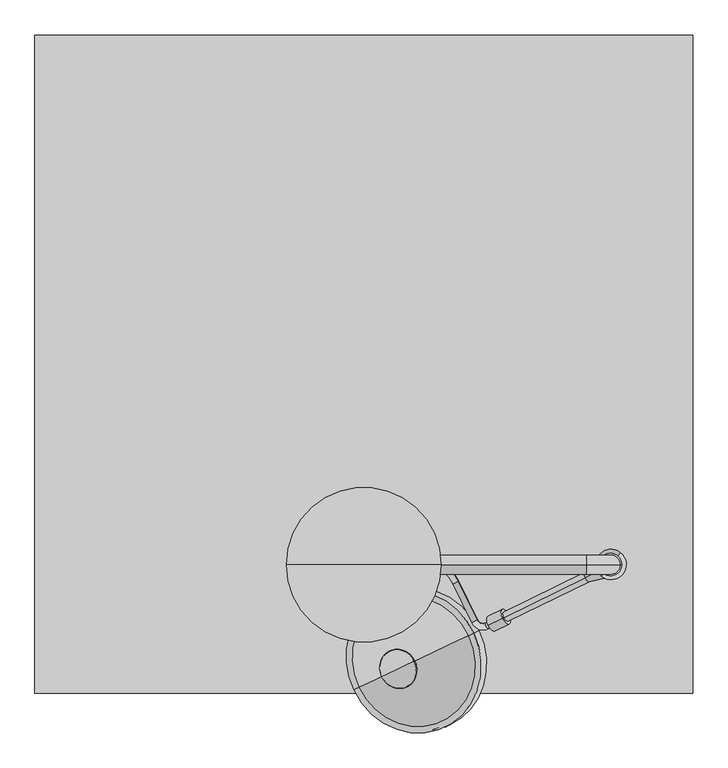
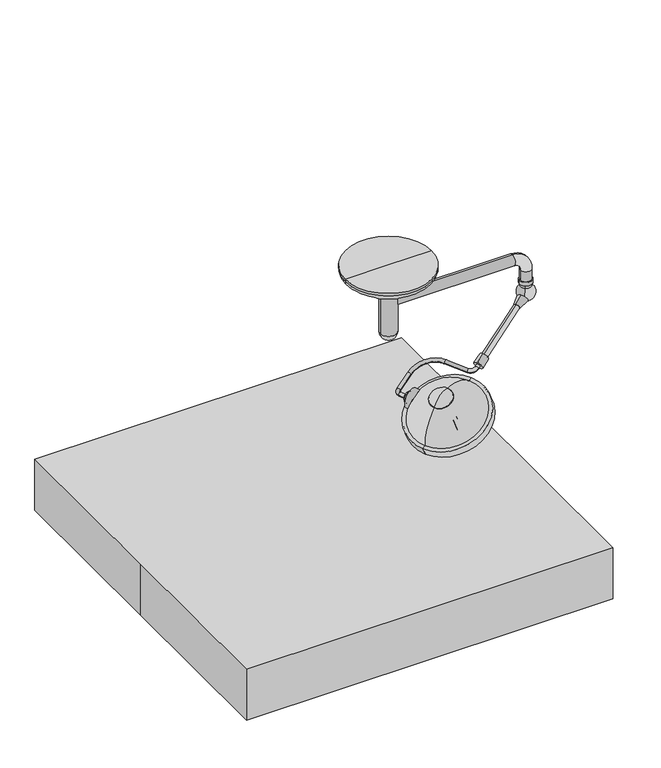
"""IFC4 building model written with IfcOpenShell, lengths in millimetres: proxy geometry, M7485 - Light, Surg, Ceiling Mtd, Dual, Equal Dia Heads : M7485 - Light, Surg, Ceiling Mtd, Dual, Equal Dia Heads."""

from ifc_helpers import new_model, si_unit, point, frame, frame_2d, origin, origin_with_axes, origin_2d, place, context, project, spatial, polyline, circle_curve, ellipse_curve, trimmed, segment, composite_curve, outline, extrude, source, transform, mapped, element, save
from ifc_brep_helpers import plane_surface, cylinder_surface, revolved_surface, advanced_brep


def specialty_equipment_7f5e032a(model_context):
    return source(origin(), model_context, "Body", "SolidModel", [
        advanced_brep(
        [(51.3241797, -908.0178384, 1699.7604265), (72.1798458, -897.8458503, 1710.0915373), (51.503984, -855.4540515, 1710.0915373), (30.6483179, -865.6260395, 1699.7604265), (56.3645035, -838.953373, 1715.2570926), (45.2298764, -816.1240043, 1715.2570926), (159.8794514, -788.4657596, 1766.5344952), (148.7448243, -765.6363908, 1766.5344952), (351.8212111, -864.410044, 1828.5211596), (372.6768772, -854.238056, 1838.8522704), (426.0821694, -1016.6675722, 1828.5211596), (446.9378356, -1006.4955842, 1838.8522704), (490.062756, -1041.9823337, 1849.1833811), (478.9281288, -1019.1529649, 1849.1833811), (557.8921303, -980.6396481, 1888.2991704), (569.0267574, -1003.4690168, 1888.2991704)],
        [
            (0, 1, circle_curve(frame((61.7520127, -902.9318443, 1704.9259819), z_axis=(0.4383711467890926, -0.8987940462991595, 0.0), x_axis=(0.8210892183528103, 0.4004719699107539, 0.4067366430758007)), 12.7)),
            (1, 0, circle_curve(frame((61.7520127, -902.9318443, 1704.9259819), z_axis=(0.4383711467890926, -0.8987940462991595, 0.0), x_axis=(0.8210892183528103, 0.4004719699107539, 0.4067366430758007)), 12.7)),
            (1, 2),
            (2, 3, circle_curve(frame((41.0761509, -860.5400455, 1704.9259819), z_axis=(0.4383711467890926, -0.8987940462991595, 0.0), x_axis=(0.8210892183528103, 0.4004719699107539, 0.4067366430758007)), 12.7)),
            (3, 0),
            (3, 2, circle_curve(frame((41.0761509, -860.5400455, 1704.9259819), z_axis=(0.4383711467890926, -0.8987940462991595, 0.0), x_axis=(0.8210892183528103, 0.4004719699107539, 0.4067366430758007)), 12.7)),
            (4, 5, circle_curve(frame((50.79719, -827.5386887, 1715.2570926), z_axis=(-0.8210892183528203, -0.40047196991073386, -0.4067366430758003), x_axis=(0.4383711467890744, -0.8987940462991688, 0.0)), 12.7)),
            (5, 3, circle_curve(frame((61.9318171, -850.3680574, 1715.2570926), z_axis=(-0.36557247320823616, -0.17830160866628347, 0.9135454576426008), x_axis=(-0.8210892183528108, -0.40047196991075346, -0.40673664307580043)), 38.1)),
            (2, 4, circle_curve(frame((61.9318171, -850.3680574, 1715.2570926), z_axis=(0.36557247320823616, 0.17830160866628347, -0.9135454576426008), x_axis=(-0.8210892183528108, -0.40047196991075346, -0.40673664307580043)), 12.7)),
            (5, 4, circle_curve(frame((50.79719, -827.5386887, 1715.2570926), z_axis=(-0.8210892183528095, -0.40047196991075623, -0.4067366430758003), x_axis=(0.43837114678909483, -0.8987940462991588, 0.0)), 12.7)),
            (4, 6),
            (6, 7, circle_curve(frame((154.3121378, -777.0510752, 1766.5344952), z_axis=(-0.8210892183528108, -0.40047196991075357, -0.40673664307580026), x_axis=(0.4383711467890922, -0.8987940462991598, 0.0)), 12.7)),
            (7, 5),
            (7, 6, circle_curve(frame((154.3121378, -777.0510752, 1766.5344952), z_axis=(-0.8210892183528108, -0.40047196991075357, -0.40673664307580026), x_axis=(0.4383711467890922, -0.8987940462991598, 0.0)), 12.7)),
            (8, 9, circle_curve(frame((362.2490441, -859.32405, 1833.686715), z_axis=(-0.4383711467890886, 0.8987940462991616, 0.0), x_axis=(-0.8210892183528131, -0.4004719699107496, -0.40673664307579993)), 12.7)),
            (9, 7, circle_curve(frame((226.6872142, -925.4419722, 1766.5344952), z_axis=(-0.36557247320823616, -0.17830160866628347, 0.9135454576426008), x_axis=(-0.43837114678909817, 0.8987940462991569, 0.0)), 177.8)),
            (6, 8, circle_curve(frame((226.6872142, -925.4419722, 1766.5344952), z_axis=(0.36557247320823616, 0.17830160866628347, -0.9135454576426008), x_axis=(-0.43837114678909817, 0.8987940462991569, 0.0)), 152.4)),
            (9, 8, circle_curve(frame((362.2490441, -859.32405, 1833.686715), z_axis=(-0.4383711467890903, 0.8987940462991608, 0.0), x_axis=(-0.8210892183528122, -0.40047196991075146, -0.40673664307579993)), 12.7)),
            (8, 10),
            (10, 11, circle_curve(frame((436.5100025, -1011.5815782, 1833.686715), z_axis=(-0.43837114678909095, 0.8987940462991604, 0.0), x_axis=(-0.8210892183528117, -0.400471969910752, -0.4067366430758)), 12.7)),
            (11, 9),
            (11, 10, circle_curve(frame((436.5100025, -1011.5815782, 1833.686715), z_axis=(-0.43837114678909095, 0.8987940462991604, 0.0), x_axis=(-0.8210892183528117, -0.400471969910752, -0.4067366430758)), 12.7)),
            (12, 13, circle_curve(frame((484.4954424, -1030.5676493, 1849.1833811), z_axis=(-0.8210892183528147, -0.40047196991074546, -0.4067366430758003), x_axis=(0.43837114678908495, -0.8987940462991637, 0.0)), 12.7)),
            (13, 11, circle_curve(frame((467.7935017, -996.3235961, 1849.1833811), z_axis=(0.36557247320823616, 0.17830160866628347, -0.9135454576426008), x_axis=(-0.8210892183528132, -0.40047196991074846, -0.40673664307580043)), 25.4)),
            (10, 12, circle_curve(frame((467.7935017, -996.3235961, 1849.1833811), z_axis=(-0.36557247320823616, -0.17830160866628347, 0.9135454576426008), x_axis=(-0.8210892183528132, -0.40047196991074846, -0.40673664307580043)), 50.8)),
            (13, 12, circle_curve(frame((484.4954424, -1030.5676493, 1849.1833811), z_axis=(-0.8210892183528112, -0.4004719699107527, -0.4067366430758003), x_axis=(0.4383711467890915, -0.8987940462991605, 0.0)), 12.7)),
            (14, 15, circle_curve(frame((563.4594439, -992.0543325, 1888.2991704), z_axis=(0.8210892183528123, 0.4004719699107504, 0.4067366430757997), x_axis=(0.4383711467890893, -0.8987940462991613, 0.0)), 12.7)),
            (15, 14, circle_curve(frame((563.4594439, -992.0543325, 1888.2991704), z_axis=(0.8210892183528123, 0.4004719699107504, 0.4067366430757997), x_axis=(0.4383711467890893, -0.8987940462991613, 0.0)), 12.7)),
            (12, 15),
            (14, 13),
        ],
        [
            plane_surface(frame((671.2712366, -605.6494555, 181.7710423), z_axis=(0.43837114678909284, -0.8987940462991596, 0.0), x_axis=(-0.36557247320823627, -0.17830160866628333, 0.9135454576426009))),
            cylinder_surface(frame((61.7520127, -902.9318443, 1704.9259819), z_axis=(0.4383711467890927, -0.8987940462991597, 0.0), x_axis=(0.8210892183528103, 0.4004719699107539, 0.4067366430758007)), 12.7),
            revolved_surface(trimmed(ellipse_curve(frame((41.0761509, -860.5400455, 1704.9259819), z_axis=(-0.4383711467890919, 0.8987940462991603, 0.0), x_axis=(0.8210892183528109, 0.4004719699107529, 0.4067366430758007)), 12.7, 12.7), [point((30.6483179, -865.6260395, 1699.7604265))], [point((51.503984, -855.4540515, 1710.0915373))], True, "CARTESIAN"), (671.451041, -553.0856686, 192.1021531), (-0.3655724732082362, -0.1783016086662835, 0.913545457642601)),
            revolved_surface(trimmed(ellipse_curve(frame((41.0761509, -860.5400455, 1704.9259819), z_axis=(-0.4383711467890919, 0.8987940462991603, 0.0), x_axis=(0.8210892183528109, 0.4004719699107529, 0.4067366430758007)), 12.7, 12.7), [point((51.503984, -855.4540515, 1710.0915373))], [point((30.6483179, -865.6260395, 1699.7604265))], True, "CARTESIAN"), (671.451041, -553.0856686, 192.1021531), (-0.3655724732082362, -0.1783016086662835, 0.913545457642601)),
            cylinder_surface(frame((50.79719, -827.5386887, 1715.2570926), z_axis=(-0.8210892183528108, -0.40047196991075357, -0.40673664307580026), x_axis=(0.4383711467890922, -0.8987940462991598, 0.0)), 12.7),
            revolved_surface(trimmed(ellipse_curve(frame((154.3121378, -777.0510752, 1766.5344952), z_axis=(0.821089218352808, 0.40047196991075945, 0.40673664307580043), x_axis=(0.4383711467890975, -0.8987940462991573, 0.0)), 12.7, 12.7), [point((148.7448243, -765.6363908, 1766.5344952))], [point((159.8794514, -788.4657596, 1766.5344952))], True, "CARTESIAN"), (836.2064381, -628.1595834, 243.3795556), (-0.3655724732082362, -0.1783016086662835, 0.913545457642601)),
            revolved_surface(trimmed(ellipse_curve(frame((154.3121378, -777.0510752, 1766.5344952), z_axis=(0.821089218352808, 0.40047196991075945, 0.40673664307580043), x_axis=(0.4383711467890975, -0.8987940462991573, 0.0)), 12.7, 12.7), [point((159.8794514, -788.4657596, 1766.5344952))], [point((148.7448243, -765.6363908, 1766.5344952))], True, "CARTESIAN"), (836.2064381, -628.1595834, 243.3795556), (-0.3655724732082362, -0.1783016086662835, 0.913545457642601)),
            cylinder_surface(frame((362.2490441, -859.32405, 1833.686715), z_axis=(-0.43837114678909106, 0.8987940462991606, 0.0), x_axis=(-0.8210892183528117, -0.400471969910752, -0.4067366430758)), 12.7),
            revolved_surface(trimmed(ellipse_curve(frame((436.5100025, -1011.5815782, 1833.686715), z_axis=(0.4383711467890874, -0.8987940462991625, 0.0), x_axis=(-0.8210892183528137, -0.400471969910748, -0.4067366430758)), 12.7, 12.7), [point((446.9378356, -1006.4955842, 1838.8522704))], [point((426.0821694, -1016.6675722, 1828.5211596))], True, "CARTESIAN"), (1077.3127256, -699.0412073, 326.0284415), (0.3655724732082362, 0.1783016086662835, -0.913545457642601)),
            revolved_surface(trimmed(ellipse_curve(frame((436.5100025, -1011.5815782, 1833.686715), z_axis=(0.4383711467890874, -0.8987940462991625, 0.0), x_axis=(-0.8210892183528137, -0.400471969910748, -0.4067366430758)), 12.7, 12.7), [point((426.0821694, -1016.6675722, 1828.5211596))], [point((446.9378356, -1006.4955842, 1838.8522704))], True, "CARTESIAN"), (1077.3127256, -699.0412073, 326.0284415), (0.3655724732082362, 0.1783016086662835, -0.913545457642601)),
            plane_surface(frame((1172.9786678, -694.7719436, 365.1442308), z_axis=(0.8210892183528122, 0.400471969910751, 0.4067366430757998), x_axis=(-0.3655724732082356, -0.1783016086662833, 0.9135454576426012))),
            cylinder_surface(frame((484.4954424, -1030.5676493, 1849.1833811), z_axis=(-0.8210892183528126, -0.4004719699107505, -0.4067366430757998), x_axis=(0.4383711467890893, -0.8987940462991613, 0.0)), 12.7),
        ],
        [
            (0, [[1, 2]]),
            (1, [[3, 4, 5, -2]]),
            (1, [[-5, 6, -3, -1]]),
            (2, [[7, 8, -4, 9]]),
            (3, [[10, -9, -6, -8]]),
            (4, [[11, 12, 13, -7]]),
            (4, [[-13, 14, -11, -10]]),
            (5, [[15, 16, -12, 17]]),
            (6, [[18, -17, -14, -16]]),
            (7, [[19, 20, 21, -15]]),
            (7, [[-21, 22, -19, -18]]),
            (8, [[23, 24, -20, 25]]),
            (9, [[26, -25, -22, -24]]),
            (10, [[27, 28]]),
            (11, [[29, -27, 30, -23]]),
            (11, [[-30, -28, -29, -26]]),
        ],
    ),
        advanced_brep(
        [(70.9853036, -912.17035, 1662.093259), (79.9012214, -931.0005545, 1662.093259), (79.9012214, -931.0005545, 1743.3108067), (70.9853036, -912.17035, 1743.3108067), (59.9841849, -888.936251, 1702.7020328), (79.9012214, -931.0005545, 1702.7020328)],
        [
            (0, 1),
            (1, 2, circle_curve(frame((79.9012214, -931.0005545, 1702.7020328), z_axis=(-0.4279431442574093, 0.903805656810734, 0.0), x_axis=(0.0, 0.0, 1.0)), 40.6087738)),
            (2, 3),
            (3, 0, circle_curve(frame((70.9853036, -912.17035, 1702.7020328), z_axis=(0.4279431442574093, -0.903805656810734, 0.0), x_axis=(0.0, 0.0, 1.0)), 40.6087738)),
            (2, 1, circle_curve(frame((79.9012214, -931.0005545, 1702.7020328), z_axis=(-0.4279431442574093, 0.903805656810734, 0.0), x_axis=(0.0, 0.0, 1.0)), 40.6087738)),
            (0, 3, circle_curve(frame((70.9853036, -912.17035, 1702.7020328), z_axis=(0.4279431442574093, -0.903805656810734, 0.0), x_axis=(0.0, 0.0, 1.0)), 40.6087738)),
            (4, 0, circle_curve(frame((83.4268503, -938.4465982, 1708.9387051), z_axis=(-0.9038056568107343, -0.42794314425740876, 0.0), x_axis=(0.4279431442574089, -0.9038056568107342, 0.0)), 55.1337385)),
            (3, 4, circle_curve(frame((83.4268503, -938.4465982, 1696.4653606), z_axis=(-0.9038056568107339, -0.42794314425740954, 0.0), x_axis=(0.4279431442574097, -0.9038056568107338, 0.0)), 55.1337385)),
            (1, 5),
            (5, 2),
        ],
        [
            cylinder_surface(frame((79.9012214, -931.0005545, 1702.7020328), z_axis=(-0.4279431442574093, 0.903805656810734, 0.0), x_axis=(0.0, 0.0, 1.0)), 40.6087738),
            revolved_surface(trimmed(ellipse_curve(frame((83.4268503, -938.4465982, 1696.4653606), z_axis=(-0.9038056568107339, -0.42794314425740954, 0.0), x_axis=(0.4279431442574097, -0.9038056568107338, 0.0)), 55.1337385, 55.1337385), [point((70.9853036, -912.17035, 1743.3108067))], [point((59.9841849, -888.936251, 1702.7020328))], True, "CARTESIAN"), (79.9012214, -931.0005545, 1702.7020328), (-0.4279431442574093, 0.903805656810734, 0.0)),
            revolved_surface(trimmed(ellipse_curve(frame((83.4268503, -938.4465982, 1696.4653606), z_axis=(-0.9038056568107339, -0.4279431442574097, 0.0), x_axis=(0.42794314425740987, -0.9038056568107338, 0.0)), 55.1337385, 55.1337385), [point((70.9853036, -912.17035, 1743.3108067))], [point((59.9841849, -888.936251, 1702.7020328))], True, "CARTESIAN"), (79.9012214, -931.0005545, 1702.7020328), (-0.4279431442574093, 0.903805656810734, 0.0)),
            plane_surface(frame((79.9012214, -931.0005545, 1702.7020328), z_axis=(0.42794314425740915, -0.9038056568107341, 0.0), x_axis=(0.0, 0.0, 1.0))),
        ],
        [
            (0, [[1, 2, 3, 4]]),
            (0, [[-3, 5, -1, 6]]),
            (1, [[7, -4, 8]]),
            (2, [[-8, -6, -7]]),
            (3, [[9, 10, -2]]),
            (3, [[-10, -9, -5]]),
        ],
    ),
        advanced_brep(
        [(198.2891405, -1170.0305938, 1882.6946884), (123.8504881, -1205.2765681, 1877.268084), (70.3964825, -1230.5865173, 1819.6927814), (200.9060117, -1168.7915308, 1880.0876662), (70.3964825, -1230.5865173, 1815.7966478), (129.8474904, -1202.4370461, 1862.3650044)],
        [
            (0, 1, circle_curve(frame((172.8421817, -1182.07948, 1682.2916913), z_axis=(0.4279431442574066, -0.9038056568107353, 0.0), x_axis=(-0.6047640271723351, -0.28634985560407467, -0.7431448254773929)), 202.3711557)),
            (1, 2, circle_curve(frame((222.0261973, -1158.7913294, 1706.5205002), z_axis=(0.42794314425740937, -0.903805656810734, 0.0), x_axis=(0.903805656810734, 0.4279431442574095, 0.0)), 202.3711557)),
            (2, 0, circle_curve(frame((134.3428115, -1200.3085555, 1851.1937349), z_axis=(-0.367610878844116, -0.17406015792256127, 0.9135454576426013), x_axis=(-0.825667552371134, -0.3909455155656486, -0.4067366430757995)), 77.4480344)),
            (0, 2, circle_curve(frame((134.3428115, -1200.3085555, 1851.1937349), z_axis=(-0.367610878844116, -0.17406015792256127, 0.9135454576426013), x_axis=(-0.825667552371134, -0.3909455155656486, -0.4067366430757995)), 77.4480344)),
            (3, 0),
            (2, 4),
            (4, 3, circle_curve(frame((135.6512471, -1199.689024, 1847.942157), z_axis=(-0.367610878844116, -0.17406015792256127, 0.9135454576426013), x_axis=(-0.825667552371134, -0.3909455155656486, -0.4067366430757995)), 79.0327347)),
            (3, 4, circle_curve(frame((135.6512471, -1199.689024, 1847.942157), z_axis=(-0.367610878844116, -0.17406015792256127, 0.9135454576426013), x_axis=(-0.825667552371134, -0.3909455155656486, -0.4067366430757995)), 79.0327347)),
            (5, 3, circle_curve(frame((221.2532479, -1159.1573133, 1596.9639329), z_axis=(-0.4279431442574066, 0.9038056568107353, 0.0), x_axis=(-0.6047640271723351, -0.28634985560407467, -0.7431448254773929)), 284.0173877)),
            (4, 5, circle_curve(frame((246.9439851, -1146.9930004, 1609.6195886), z_axis=(-0.42794314425740937, 0.903805656810734, 0.0), x_axis=(0.903805656810734, 0.4279431442574095, 0.0)), 284.0173877)),
        ],
        [
            revolved_surface(trimmed(ellipse_curve(frame((222.0261973, -1158.7913294, 1706.5205002), z_axis=(0.42794314425740937, -0.903805656810734, 0.0), x_axis=(0.903805656810734, 0.4279431442574095, 0.0)), 202.3711557, 202.3711557), [point((123.8504881, -1205.2765681, 1877.268084))], [point((70.3964825, -1230.5865173, 1819.6927814))], True, "CARTESIAN"), (169.8512246, -1183.495669, 1762.9521965), (0.367610878844116, 0.17406015792256127, -0.9135454576426013)),
            revolved_surface(trimmed(ellipse_curve(frame((222.0261973, -1158.7913294, 1706.5205002), z_axis=(0.42794314425740965, -0.9038056568107342, 0.0), x_axis=(0.903805656810734, 0.4279431442574096, 0.0)), 202.3711557, 202.3711557), [point((123.8504881, -1205.2765681, 1877.268084))], [point((70.3964825, -1230.5865173, 1819.6927814))], True, "CARTESIAN"), (169.8512246, -1183.495669, 1762.9521965), (0.367610878844116, 0.17406015792256127, -0.9135454576426013)),
            revolved_surface(polyline([(70.3964825, -1230.5865173, 1819.6927814), (70.3964825, -1230.5865173, 1815.7966478)]), (169.8512246, -1183.495669, 1762.9521965), (0.367610878844116, 0.17406015792256127, -0.9135454576426013)),
            revolved_surface(trimmed(ellipse_curve(frame((246.9439851, -1146.9930004, 1609.6195886), z_axis=(-0.42794314425740937, 0.903805656810734, 0.0), x_axis=(0.903805656810734, 0.4279431442574095, 0.0)), 284.0173877, 284.0173877), [point((70.3964825, -1230.5865173, 1815.7966478))], [point((129.8474904, -1202.4370461, 1862.3650044))], True, "CARTESIAN"), (169.8512246, -1183.495669, 1762.9521965), (0.367610878844116, 0.17406015792256127, -0.9135454576426013)),
            revolved_surface(trimmed(ellipse_curve(frame((246.9439851, -1146.9930004, 1609.6195886), z_axis=(-0.42794314425740965, 0.9038056568107342, 0.0), x_axis=(0.903805656810734, 0.4279431442574096, 0.0)), 284.0173877, 284.0173877), [point((70.3964825, -1230.5865173, 1815.7966478))], [point((129.8474904, -1202.4370461, 1862.3650044))], True, "CARTESIAN"), (169.8512246, -1183.495669, 1762.9521965), (0.367610878844116, 0.17406015792256127, -0.9135454576426013)),
        ],
        [
            (0, [[1, 2, 3]]),
            (1, [[-2, -1, 4]]),
            (2, [[5, -3, 6, 7]]),
            (2, [[-6, -4, -5, 8]]),
            (3, [[9, -7, 10]]),
            (4, [[-10, -8, -9]]),
        ],
    ),
        advanced_brep(
        [(266.4821549, -1137.741868, 1522.8158117), (255.996177, -1142.7068761, 1517.6502563), (276.9681328, -1132.77686, 1527.9813671), (263.0629437, -1139.3608311, 1507.6425198), (271.0121339, -1135.5969672, 1511.5584142), (278.9613242, -1131.8331033, 1515.4743086)],
        [
            (0, 1),
            (1, 2, circle_curve(frame((266.4821549, -1137.741868, 1522.8158117), z_axis=(-0.3676108788441159, -0.1740601579225613, 0.9135454576426013), x_axis=(0.825667552371134, 0.3909455155656486, 0.40673664307579943)), 12.7)),
            (2, 0),
            (2, 1, circle_curve(frame((266.4821549, -1137.741868, 1522.8158117), z_axis=(-0.3676108788441159, -0.1740601579225613, 0.9135454576426013), x_axis=(0.825667552371134, 0.3909455155656486, 0.40673664307579943)), 12.7)),
            (3, 4),
            (4, 5),
            (5, 3, circle_curve(frame((271.0121339, -1135.5969672, 1511.5584142), z_axis=(0.3676108788441159, 0.1740601579225613, -0.9135454576426013), x_axis=(0.825667552371134, 0.3909455155656486, 0.40673664307579943)), 9.6275919)),
            (3, 5, circle_curve(frame((271.0121339, -1135.5969672, 1511.5584142), z_axis=(0.3676108788441159, 0.1740601579225613, -0.9135454576426013), x_axis=(0.825667552371134, 0.3909455155656486, 0.40673664307579943)), 9.6275919)),
            (1, 3),
            (5, 2),
        ],
        [
            plane_surface(frame((266.4821549, -1137.741868, 1522.8158117), z_axis=(-0.367610878844116, -0.17406015792256121, 0.9135454576426014), x_axis=(0.8256675523711339, 0.39094551556564855, 0.4067366430757994))),
            plane_surface(frame((271.0121339, -1135.5969672, 1511.5584142), z_axis=(0.367610878844116, 0.17406015792256121, -0.9135454576426014), x_axis=(0.8256675523711339, 0.39094551556564855, 0.4067366430757994))),
            revolved_surface(polyline([(278.9613242, -1131.8331033, 1515.4743086), (276.9681328, -1132.77686, 1527.9813671)]), (229.1328896, -1155.4263801, 1615.6320302), (-0.3676108788441159, -0.1740601579225613, 0.9135454576426013)),
        ],
        [
            (0, [[1, 2, 3]]),
            (0, [[-3, 4, -1]]),
            (1, [[5, 6, 7]]),
            (1, [[-6, -5, 8]]),
            (2, [[9, -7, 10, -2]]),
            (2, [[-10, -8, -9, -4]]),
        ],
    ),
        advanced_brep(
        [(229.1328896, -1155.4263801, 1615.6320302), (213.4039227, -1162.8738921, 1607.8836971), (244.8618565, -1147.978868, 1623.3803632), (250.753188, -1145.1893801, 1515.0674786), (266.4821549, -1137.741868, 1522.8158117), (282.2111217, -1130.2943559, 1530.5641447)],
        [
            (0, 1),
            (1, 2, circle_curve(frame((229.1328896, -1155.4263801, 1615.6320302), z_axis=(-0.3676108788441159, -0.1740601579225613, 0.9135454576426013), x_axis=(0.825667552371134, 0.3909455155656486, 0.40673664307579943)), 19.05)),
            (2, 0),
            (2, 1, circle_curve(frame((229.1328896, -1155.4263801, 1615.6320302), z_axis=(-0.3676108788441159, -0.1740601579225613, 0.9135454576426013), x_axis=(0.825667552371134, 0.3909455155656486, 0.40673664307579943)), 19.05)),
            (3, 4),
            (4, 5),
            (5, 3, circle_curve(frame((266.4821549, -1137.741868, 1522.8158117), z_axis=(0.3676108788441159, 0.1740601579225613, -0.9135454576426013), x_axis=(0.825667552371134, 0.3909455155656486, 0.40673664307579943)), 19.05)),
            (3, 5, circle_curve(frame((266.4821549, -1137.741868, 1522.8158117), z_axis=(0.3676108788441159, 0.1740601579225613, -0.9135454576426013), x_axis=(0.825667552371134, 0.3909455155656486, 0.40673664307579943)), 19.05)),
            (1, 3),
            (5, 2),
        ],
        [
            plane_surface(frame((229.1328896, -1155.4263801, 1615.6320302), z_axis=(-0.367610878844116, -0.17406015792256121, 0.9135454576426014), x_axis=(0.8256675523711339, 0.39094551556564855, 0.4067366430757994))),
            plane_surface(frame((266.4821549, -1137.741868, 1522.8158117), z_axis=(0.367610878844116, 0.17406015792256121, -0.9135454576426014), x_axis=(0.8256675523711339, 0.39094551556564855, 0.4067366430757994))),
            cylinder_surface(frame((229.1328896, -1155.4263801, 1615.6320302), z_axis=(-0.3676108788441159, -0.1740601579225613, 0.9135454576426013), x_axis=(0.825667552371134, 0.3909455155656486, 0.40673664307579943)), 19.05),
        ],
        [
            (0, [[1, 2, 3]]),
            (0, [[-3, 4, -1]]),
            (1, [[5, 6, 7]]),
            (1, [[-6, -5, 8]]),
            (2, [[9, -7, 10, -2]]),
            (2, [[-10, -8, -9, -4]]),
        ],
    ),
        advanced_brep(
        [(222.1299023, -1158.7422261, 1633.0350712), (185.4289796, -1176.1197542, 1614.9556274), (258.830825, -1141.3646979, 1651.1145149), (192.4319669, -1172.8039082, 1597.5525864), (229.1328896, -1155.4263801, 1615.6320302), (265.8338123, -1138.0488519, 1633.711474)],
        [
            (0, 1),
            (1, 2, circle_curve(frame((222.1299023, -1158.7422261, 1633.0350712), z_axis=(-0.36761087884411536, -0.17406015792256102, 0.9135454576426016), x_axis=(0.8256675523711342, 0.3909455155656487, 0.4067366430757988)), 44.45)),
            (2, 0),
            (2, 1, circle_curve(frame((222.1299023, -1158.7422261, 1633.0350712), z_axis=(-0.36761087884411536, -0.17406015792256102, 0.9135454576426016), x_axis=(0.8256675523711342, 0.3909455155656487, 0.4067366430757988)), 44.45)),
            (3, 4),
            (4, 5),
            (5, 3, circle_curve(frame((229.1328896, -1155.4263801, 1615.6320302), z_axis=(0.36761087884411536, 0.17406015792256102, -0.9135454576426016), x_axis=(0.8256675523711342, 0.3909455155656487, 0.4067366430757988)), 44.45)),
            (3, 5, circle_curve(frame((229.1328896, -1155.4263801, 1615.6320302), z_axis=(0.36761087884411536, 0.17406015792256102, -0.9135454576426016), x_axis=(0.8256675523711342, 0.3909455155656487, 0.4067366430757988)), 44.45)),
            (1, 3),
            (5, 2),
        ],
        [
            plane_surface(frame((222.1299023, -1158.7422261, 1633.0350712), z_axis=(-0.3676108788441154, -0.17406015792256094, 0.9135454576426016), x_axis=(0.8256675523711341, 0.39094551556564866, 0.40673664307579876))),
            plane_surface(frame((229.1328896, -1155.4263801, 1615.6320302), z_axis=(0.3676108788441154, 0.17406015792256094, -0.9135454576426016), x_axis=(0.8256675523711341, 0.39094551556564866, 0.40673664307579876))),
            cylinder_surface(frame((222.1299023, -1158.7422261, 1633.0350712), z_axis=(-0.36761087884411536, -0.17406015792256102, 0.9135454576426016), x_axis=(0.8256675523711342, 0.3909455155656487, 0.4067366430757988)), 44.45),
        ],
        [
            (0, [[1, 2, 3]]),
            (0, [[-3, 4, -1]]),
            (1, [[5, 6, 7]]),
            (1, [[-6, -5, 8]]),
            (2, [[9, -7, 10, -2]]),
            (2, [[-10, -8, -9, -4]]),
        ],
    ),
        advanced_brep(
        [(217.8648709, -1160.7616768, 1643.6340505), (170.6779703, -1183.104213, 1620.3890514), (265.0517715, -1138.4191406, 1666.8790497), (179.2080332, -1179.0653116, 1611.8910927), (222.1299023, -1158.7422261, 1633.0350712), (265.0517715, -1138.4191406, 1654.1790497)],
        [
            (0, 1),
            (1, 2, circle_curve(frame((217.8648709, -1160.7616768, 1643.6340505), z_axis=(-0.36761087884411614, -0.1740601579225614, 0.9135454576426012), x_axis=(0.8256675523711339, 0.39094551556564855, 0.4067366430757997)), 57.15)),
            (2, 0),
            (2, 1, circle_curve(frame((217.8648709, -1160.7616768, 1643.6340505), z_axis=(-0.36761087884411614, -0.1740601579225614, 0.9135454576426012), x_axis=(0.8256675523711339, 0.39094551556564855, 0.4067366430757997)), 57.15)),
            (3, 4),
            (4, 5),
            (5, 3, circle_curve(frame((222.1299023, -1158.7422261, 1633.0350712), z_axis=(0.36761087884411614, 0.1740601579225614, -0.9135454576426012), x_axis=(0.8256675523711339, 0.39094551556564855, 0.4067366430757997)), 51.9844446)),
            (3, 5, circle_curve(frame((222.1299023, -1158.7422261, 1633.0350712), z_axis=(0.36761087884411614, 0.1740601579225614, -0.9135454576426012), x_axis=(0.8256675523711339, 0.39094551556564855, 0.4067366430757997)), 51.9844446)),
            (1, 3),
            (5, 2),
        ],
        [
            plane_surface(frame((217.8648709, -1160.7616768, 1643.6340505), z_axis=(-0.36761087884411625, -0.17406015792256133, 0.9135454576426013), x_axis=(0.8256675523711338, 0.3909455155656485, 0.40673664307579965))),
            plane_surface(frame((222.1299023, -1158.7422261, 1633.0350712), z_axis=(0.36761087884411625, 0.17406015792256133, -0.9135454576426013), x_axis=(0.8256675523711338, 0.3909455155656485, 0.40673664307579965))),
            revolved_surface(polyline([(265.0517715, -1138.4191406, 1654.1790497), (265.0517715, -1138.4191406, 1666.8790497)]), (217.8648709, -1160.7616768, 1643.6340505), (-0.36761087884411614, -0.1740601579225614, 0.9135454576426012)),
        ],
        [
            (0, [[1, 2, 3]]),
            (0, [[-3, 4, -1]]),
            (1, [[5, 6, 7]]),
            (1, [[-6, -5, 8]]),
            (2, [[9, -7, 10, -2]]),
            (2, [[-10, -8, -9, -4]]),
        ],
    ),
        extrude(outline(composite_curve([segment(trimmed(circle_curve(frame_2d((0.0, 69.9387006)), 69.9387006), [point((-25.1937137, 4.6953206))], [point((31.6273953, 132.3176211))], False, "CARTESIAN"), True, "CONTINUOUS"), segment(polyline([(31.6273953, 132.3176211), (-25.1937137, 4.6953206)]), True, "CONTINUOUS")], self_intersect=False)), frame((180.69854, -976.5021254, 1699.0600142), z_axis=(-0.42794314425740915, 0.9038056568107341, 0.0), x_axis=(0.0, 0.0, -1.0)), (0.0, 0.0, 1.0), 84.2600986),
        advanced_brep(
        [(411.8184564, -1068.9265498, 1801.7370584), (129.8408016, -1202.4402132, 1862.3816266), (-18.1066381, -1272.4918798, 1589.9492884), (406.0906916, -1071.6385905, 1798.9154726), (-12.3788733, -1269.7798391, 1592.7708742), (132.17953, -1201.3328482, 1856.5696802)],
        [
            (0, 1, circle_curve(frame((226.1466857, -1156.8403184, 1577.7194701), z_axis=(0.4279431442574066, -0.9038056568107353, 0.0), x_axis=(-0.6047640271723351, -0.2863498556040747, -0.7431448254773931)), 303.9518334)),
            (1, 2, circle_curve(frame((256.5953432, -1142.4231767, 1592.718951), z_axis=(0.4279431442574095, -0.903805656810734, 0.0), x_axis=(0.9038056568107341, 0.4279431442574096, 0.0)), 303.9518334)),
            (2, 0, circle_curve(frame((196.8559092, -1170.7092148, 1695.8431734), z_axis=(-0.3676108788441161, -0.17406015792256135, 0.9135454576426013), x_axis=(-0.825667552371134, -0.3909455155656486, -0.4067366430757996)), 260.35)),
            (0, 2, circle_curve(frame((196.8559092, -1170.7092148, 1695.8431734), z_axis=(-0.3676108788441161, -0.17406015792256135, 0.9135454576426013), x_axis=(-0.825667552371134, -0.3909455155656486, -0.4067366430757996)), 260.35)),
            (3, 0),
            (2, 4),
            (4, 3, circle_curve(frame((196.8559092, -1170.7092148, 1695.8431734), z_axis=(-0.3676108788441161, -0.17406015792256135, 0.9135454576426013), x_axis=(-0.825667552371134, -0.3909455155656486, -0.4067366430757996)), 253.412868)),
            (3, 4, circle_curve(frame((196.8559092, -1170.7092148, 1695.8431734), z_axis=(-0.3676108788441161, -0.17406015792256135, 0.9135454576426013), x_axis=(-0.825667552371134, -0.3909455155656486, -0.4067366430757996)), 253.412868)),
            (5, 3, circle_curve(frame((226.1466857, -1156.8403184, 1577.7194701), z_axis=(-0.4279431442574066, 0.9038056568107353, 0.0), x_axis=(-0.6047640271723351, -0.2863498556040747, -0.7431448254773931)), 297.6018334)),
            (4, 5, circle_curve(frame((256.5953432, -1142.4231767, 1592.718951), z_axis=(-0.4279431442574095, 0.903805656810734, 0.0), x_axis=(0.9038056568107341, 0.4279431442574096, 0.0)), 297.6018334)),
        ],
        [
            revolved_surface(trimmed(ellipse_curve(frame((256.5953432, -1142.4231767, 1592.718951), z_axis=(0.4279431442574095, -0.903805656810734, 0.0), x_axis=(0.9038056568107341, 0.4279431442574096, 0.0)), 303.9518334, 303.9518334), [point((129.8408016, -1202.4402132, 1862.3816266))], [point((-18.1066381, -1272.4918798, 1589.9492884))], True, "CARTESIAN"), (196.8559092, -1170.7092148, 1695.8431734), (0.3676108788441161, 0.17406015792256135, -0.9135454576426013)),
            revolved_surface(trimmed(ellipse_curve(frame((256.5953432, -1142.4231767, 1592.718951), z_axis=(0.4279431442574094, -0.9038056568107338, 0.0), x_axis=(0.9038056568107341, 0.42794314425740954, 0.0)), 303.9518334, 303.9518334), [point((129.8408016, -1202.4402132, 1862.3816266))], [point((-18.1066381, -1272.4918798, 1589.9492884))], True, "CARTESIAN"), (196.8559092, -1170.7092148, 1695.8431734), (0.3676108788441161, 0.17406015792256135, -0.9135454576426013)),
            plane_surface(frame((196.8559092, -1170.7092148, 1695.8431734), z_axis=(0.36761087884411614, 0.17406015792256127, -0.9135454576426014), x_axis=(-0.8256675523711339, -0.39094551556564855, -0.40673664307579954))),
            revolved_surface(trimmed(ellipse_curve(frame((256.5953432, -1142.4231767, 1592.718951), z_axis=(-0.4279431442574095, 0.903805656810734, 0.0), x_axis=(0.9038056568107341, 0.4279431442574096, 0.0)), 297.6018334, 297.6018334), [point((-12.3788733, -1269.7798391, 1592.7708742))], [point((132.17953, -1201.3328482, 1856.5696802))], True, "CARTESIAN"), (196.8559092, -1170.7092148, 1695.8431734), (0.3676108788441161, 0.17406015792256135, -0.9135454576426013)),
            revolved_surface(trimmed(ellipse_curve(frame((256.5953432, -1142.4231767, 1592.718951), z_axis=(-0.4279431442574094, 0.9038056568107338, 0.0), x_axis=(0.9038056568107341, 0.42794314425740954, 0.0)), 297.6018334, 297.6018334), [point((-12.3788733, -1269.7798391, 1592.7708742))], [point((132.17953, -1201.3328482, 1856.5696802))], True, "CARTESIAN"), (196.8559092, -1170.7092148, 1695.8431734), (0.3676108788441161, 0.17406015792256135, -0.9135454576426013)),
        ],
        [
            (0, [[1, 2, 3]]),
            (1, [[-2, -1, 4]]),
            (2, [[5, -3, 6, 7]]),
            (2, [[-6, -4, -5, 8]]),
            (3, [[9, -7, 10]]),
            (4, [[-10, -8, -9]]),
        ],
    ),
        advanced_brep(
        [(453.799374, -1049.0489957, 1759.8590463), (432.7904123, -1058.9965337, 1812.0681692), (-39.0785939, -1282.4218959, 1579.6181777), (-18.0696322, -1272.4743578, 1527.4090547), (448.556385, -1051.5314997, 1757.2762686), (-12.8266432, -1269.9918538, 1529.9918324), (429.8817524, -1060.3737557, 1803.6843778), (-31.5012759, -1278.8341098, 1576.3999417), (199.1902382, -1169.6039328, 1690.0421598), (196.8559092, -1170.7092148, 1695.8431734)],
        [
            (0, 1),
            (1, 2, circle_curve(frame((196.8559092, -1170.7092148, 1695.8431734), z_axis=(0.3676108788441158, 0.1740601579225612, -0.9135454576426014), x_axis=(-0.8256675523711341, -0.39094551556564866, -0.4067366430757993)), 285.75)),
            (2, 3),
            (3, 0, circle_curve(frame((217.8648709, -1160.7616768, 1643.6340505), z_axis=(-0.3676108788441158, -0.1740601579225612, 0.9135454576426014), x_axis=(-0.8256675523711341, -0.39094551556564866, -0.4067366430757993)), 285.75)),
            (2, 1, circle_curve(frame((196.8559092, -1170.7092148, 1695.8431734), z_axis=(0.3676108788441158, 0.1740601579225612, -0.9135454576426014), x_axis=(-0.8256675523711341, -0.39094551556564866, -0.4067366430757993)), 285.75)),
            (0, 3, circle_curve(frame((217.8648709, -1160.7616768, 1643.6340505), z_axis=(-0.3676108788441158, -0.1740601579225612, 0.9135454576426014), x_axis=(-0.8256675523711341, -0.39094551556564866, -0.4067366430757993)), 285.75)),
            (4, 0),
            (3, 5),
            (5, 4, circle_curve(frame((217.8648709, -1160.7616768, 1643.6340505), z_axis=(-0.3676108788441158, -0.1740601579225612, 0.9135454576426014), x_axis=(-0.8256675523711341, -0.39094551556564866, -0.4067366430757993)), 279.4)),
            (4, 5, circle_curve(frame((217.8648709, -1160.7616768, 1643.6340505), z_axis=(-0.3676108788441158, -0.1740601579225612, 0.9135454576426014), x_axis=(-0.8256675523711341, -0.39094551556564866, -0.4067366430757993)), 279.4)),
            (6, 4),
            (5, 7),
            (7, 6, circle_curve(frame((199.1902382, -1169.6039328, 1690.0421598), z_axis=(-0.3676108788441158, -0.1740601579225612, 0.9135454576426014), x_axis=(-0.8256675523711341, -0.39094551556564866, -0.4067366430757993)), 279.4)),
            (6, 7, circle_curve(frame((199.1902382, -1169.6039328, 1690.0421598), z_axis=(-0.3676108788441158, -0.1740601579225612, 0.9135454576426014), x_axis=(-0.8256675523711341, -0.39094551556564866, -0.4067366430757993)), 279.4)),
            (8, 6),
            (7, 8),
            (1, 9),
            (9, 2),
        ],
        [
            cylinder_surface(frame((217.8648709, -1160.7616768, 1643.6340505), z_axis=(0.3676108788441158, 0.1740601579225612, -0.9135454576426014), x_axis=(-0.8256675523711341, -0.39094551556564866, -0.4067366430757993)), 285.75),
            plane_surface(frame((217.8648709, -1160.7616768, 1643.6340505), z_axis=(0.3676108788441158, 0.17406015792256113, -0.9135454576426014), x_axis=(-0.8256675523711339, -0.39094551556564855, -0.4067366430757992))),
            revolved_surface(polyline([(-12.826643216696848, -1269.991853841562, 1529.9918323853622), (-31.501275901114123, -1278.8341098825588, 1576.3999417308632)]), (217.8648709, -1160.7616768, 1643.6340505), (0.3676108788441158, 0.1740601579225612, -0.9135454576426014)),
            plane_surface(frame((199.1902382, -1169.6039328, 1690.0421598), z_axis=(0.3676108788441158, 0.17406015792256113, -0.9135454576426014), x_axis=(-0.8256675523711339, -0.39094551556564855, -0.4067366430757992))),
            plane_surface(frame((196.8559092, -1170.7092148, 1695.8431734), z_axis=(-0.3676108788441158, -0.17406015792256113, 0.9135454576426014), x_axis=(-0.8256675523711339, -0.39094551556564855, -0.4067366430757992))),
        ],
        [
            (0, [[1, 2, 3, 4]]),
            (0, [[-3, 5, -1, 6]]),
            (1, [[7, -4, 8, 9]]),
            (1, [[-8, -6, -7, 10]]),
            (2, [[11, -9, 12, 13]]),
            (2, [[-12, -10, -11, 14]]),
            (3, [[15, -13, 16]]),
            (3, [[-16, -14, -15]]),
            (4, [[17, 18, -2]]),
            (4, [[-18, -17, -5]]),
        ],
    ),
        advanced_brep(
        [(571.2157425, -988.2713329, 1857.3919398), (559.1556073, -994.1534538, 1886.167212), (547.0954721, -1000.0355748, 1914.9424843), (514.3170471, -1016.0226809, 1827.8720542), (490.1967767, -1027.7869228, 1885.4225987), (502.2569119, -1021.9048018, 1856.6473264)],
        [
            (0, 1),
            (1, 2),
            (2, 0, circle_curve(frame((559.1556073, -994.1534538, 1886.167212), z_axis=(0.8145840431031092, 0.39729918394713865, 0.42261826174069883), x_axis=(-0.3798467775098406, -0.18526365205328194, 0.9063077870366504)), 31.75)),
            (0, 2, circle_curve(frame((559.1556073, -994.1534538, 1886.167212), z_axis=(0.8145840431031092, 0.39729918394713865, 0.42261826174069883), x_axis=(-0.3798467775098406, -0.18526365205328194, 0.9063077870366504)), 31.75)),
            (3, 0),
            (2, 4),
            (4, 3, circle_curve(frame((502.2569119, -1021.9048018, 1856.6473264), z_axis=(0.8145840431031092, 0.39729918394713865, 0.42261826174069883), x_axis=(-0.3798467775098406, -0.18526365205328194, 0.9063077870366504)), 31.75)),
            (3, 4, circle_curve(frame((502.2569119, -1021.9048018, 1856.6473264), z_axis=(0.8145840431031092, 0.39729918394713865, 0.42261826174069883), x_axis=(-0.3798467775098406, -0.18526365205328194, 0.9063077870366504)), 31.75)),
            (5, 3),
            (4, 5),
        ],
        [
            plane_surface(frame((559.1556073, -994.1534538, 1886.167212), z_axis=(0.8145840431031093, 0.39729918394713865, 0.42261826174069883), x_axis=(-0.3798467775098406, -0.18526365205328194, 0.9063077870366504))),
            cylinder_surface(frame((559.1556073, -994.1534538, 1886.167212), z_axis=(-0.8145840431031092, -0.39729918394713865, -0.42261826174069883), x_axis=(-0.3798467775098406, -0.18526365205328194, 0.9063077870366504)), 31.75),
            plane_surface(frame((502.2569119, -1021.9048018, 1856.6473264), z_axis=(-0.8145840431031093, -0.39729918394713865, -0.42261826174069883), x_axis=(-0.3798467775098406, -0.18526365205328194, 0.9063077870366504))),
        ],
        [
            (0, [[1, 2, 3]]),
            (0, [[-2, -1, 4]]),
            (1, [[5, -3, 6, 7]]),
            (1, [[-6, -4, -5, 8]]),
            (2, [[9, -7, 10]]),
            (2, [[-10, -8, -9]]),
        ],
    ),
        extrude(outline(composite_curve([segment(trimmed(circle_curve(origin_2d(), 20.2288163), [point((0.0, 20.2288164))], [point((0.0, -20.2288163))], False, "CARTESIAN"), True, "CONTINUOUS"), segment(trimmed(circle_curve(origin_2d(), 20.2288163), [point((0.0, -20.2288163))], [point((0.0, 20.2288164))], False, "CARTESIAN"), True, "CONTINUOUS")], self_intersect=False)), frame((559.1556073, -994.1534538, 1886.167212), z_axis=(0.8145840431031093, 0.3972991839471386, 0.4226182617406987), x_axis=(-0.43837114678908984, 0.8987940462991609, 0.0)), (0.0, 0.0, 1.0), 393.7),
        advanced_brep(
        [(940.9549717, -807.9374615, 2081.4066897), (928.0978809, -814.2082837, 2115.1067436), (953.8120625, -801.6666393, 2047.7066358), (872.3231351, -841.4114448, 2072.3001347), (879.8573451, -837.7367651, 2052.5520217), (887.391555, -834.0620854, 2032.8039086)],
        [
            (0, 1),
            (1, 2, circle_curve(frame((940.9549717, -807.9374615, 2081.4066897), z_axis=(0.827344281872535, 0.4035227682328693, 0.3907311284892741), x_axis=(0.35118681198991203, 0.17128525288203836, -0.9205048534524403)), 36.6104033)),
            (2, 0),
            (2, 1, circle_curve(frame((940.9549717, -807.9374615, 2081.4066897), z_axis=(0.827344281872535, 0.4035227682328693, 0.3907311284892741), x_axis=(0.35118681198991203, 0.17128525288203836, -0.9205048534524403)), 36.6104033)),
            (3, 4),
            (4, 5),
            (5, 3, circle_curve(frame((879.8573451, -837.7367651, 2052.5520217), z_axis=(-0.827344281872535, -0.4035227682328693, -0.3907311284892741), x_axis=(0.35118681198991203, 0.17128525288203836, -0.9205048534524403)), 21.4535676)),
            (3, 5, circle_curve(frame((879.8573451, -837.7367651, 2052.5520217), z_axis=(-0.827344281872535, -0.4035227682328693, -0.3907311284892741), x_axis=(0.35118681198991203, 0.17128525288203836, -0.9205048534524403)), 21.4535676)),
            (1, 3),
            (5, 2),
        ],
        [
            plane_surface(frame((940.9549717, -807.9374615, 2081.4066897), z_axis=(0.827344281872535, 0.4035227682328693, 0.39073112848927416), x_axis=(0.35118681198991203, 0.17128525288203836, -0.9205048534524403))),
            plane_surface(frame((879.8573451, -837.7367651, 2052.5520217), z_axis=(-0.827344281872535, -0.4035227682328693, -0.39073112848927416), x_axis=(0.35118681198991203, 0.17128525288203836, -0.9205048534524403))),
            revolved_surface(polyline([(887.391555, -834.0620854, 2032.8039086), (953.8120625, -801.6666393, 2047.7066358)]), (921.8864346, -817.2378085, 2072.401163), (0.827344281872535, 0.4035227682328693, 0.3907311284892741)),
        ],
        [
            (0, [[1, 2, 3]]),
            (0, [[-3, 4, -1]]),
            (1, [[5, 6, 7]]),
            (1, [[-6, -5, 8]]),
            (2, [[9, -7, 10, -2]]),
            (2, [[-10, -8, -9, -4]]),
        ],
    ),
        advanced_brep(
        [(973.5341458, -788.4695301, 2175.962195), (997.5112527, -758.860269, 2175.962195), (949.5570389, -818.0787912, 2175.962195), (997.5112527, -758.860269, 2150.1869575), (973.5341458, -788.4695301, 2044.1286543), (949.5570389, -818.0787912, 2150.1869575)],
        [
            (0, 1),
            (1, 2, circle_curve(frame((973.5341458, -788.4695301, 2175.962195), z_axis=(0.0, 0.0, 1.0), x_axis=(-0.6293203910498301, -0.777145961456977, 0.0)), 38.1)),
            (2, 0),
            (2, 1, circle_curve(frame((973.5341458, -788.4695301, 2175.962195), z_axis=(0.0, 0.0, 1.0), x_axis=(-0.6293203910498301, -0.777145961456977, 0.0)), 38.1)),
            (3, 4, circle_curve(frame((973.5341458, -788.4695301, 2104.0012588), z_axis=(-0.7771459614569791, 0.6293203910498274, 0.0), x_axis=(0.6293203910498274, 0.7771459614569791, 0.0)), 59.8726045)),
            (4, 5, circle_curve(frame((973.5341458, -788.4695301, 2104.0012588), z_axis=(-0.7771459614569771, 0.62932039104983, 0.0), x_axis=(-0.62932039104983, -0.7771459614569771, 0.0)), 59.8726045)),
            (5, 3, circle_curve(frame((973.5341458, -788.4695301, 2150.1869575), z_axis=(0.0, 0.0, -1.0), x_axis=(-0.6293203910498301, -0.777145961456977, 0.0)), 38.1)),
            (3, 5, circle_curve(frame((973.5341458, -788.4695301, 2150.1869575), z_axis=(0.0, 0.0, -1.0), x_axis=(-0.6293203910498301, -0.777145961456977, 0.0)), 38.1)),
            (1, 3),
            (5, 2),
        ],
        [
            plane_surface(frame((973.5341458, -788.4695301, 2175.962195), z_axis=(0.0, 0.0, 1.0000000000000002), x_axis=(-0.6293203910498301, -0.777145961456977, 0.0))),
            revolved_surface(trimmed(ellipse_curve(frame((973.5341458, -788.4695301, 2104.0012588), z_axis=(-0.7771459614569771, 0.62932039104983, 0.0), x_axis=(-0.62932039104983, -0.7771459614569771, 0.0)), 59.8726045, 59.8726045), [point((973.5341458, -788.4695301, 2044.1286543))], [point((949.5570389, -818.0787912, 2150.1869575))], True, "CARTESIAN"), (973.5341458, -788.4695301, 2175.962195), (0.0, 0.0, 1.0)),
            cylinder_surface(frame((973.5341458, -788.4695301, 2175.962195), z_axis=(0.0, 0.0, 1.0), x_axis=(-0.6293203910498301, -0.777145961456977, 0.0)), 38.1),
        ],
        [
            (0, [[1, 2, 3]]),
            (0, [[-3, 4, -1]]),
            (1, [[5, 6, 7]]),
            (1, [[-6, -5, 8]]),
            (2, [[9, -7, 10, -2]]),
            (2, [[-10, -8, -9, -4]]),
        ],
    ),
        advanced_brep(
        [(927.1, -789.691789, 2175.962195), (971.55, -789.691789, 2175.962195), (1016.0, -789.691789, 2175.962195), (927.1, -789.691789, 2201.362195), (1016.0, -789.691789, 2201.362195), (971.55, -789.691789, 2201.362195)],
        [
            (0, 1),
            (1, 2),
            (2, 0, circle_curve(frame((971.55, -789.691789, 2175.962195), z_axis=(0.0, 0.0, -1.0), x_axis=(1.0, 0.0, 0.0)), 44.45)),
            (0, 2, circle_curve(frame((971.55, -789.691789, 2175.962195), z_axis=(0.0, 0.0, -1.0), x_axis=(1.0, 0.0, 0.0)), 44.45)),
            (3, 0),
            (2, 4),
            (4, 3, circle_curve(frame((971.55, -789.691789, 2201.362195), z_axis=(0.0, 0.0, -1.0), x_axis=(1.0, 0.0, 0.0)), 44.45)),
            (3, 4, circle_curve(frame((971.55, -789.691789, 2201.362195), z_axis=(0.0, 0.0, -1.0), x_axis=(1.0, 0.0, 0.0)), 44.45)),
            (5, 3),
            (4, 5),
        ],
        [
            plane_surface(frame((971.55, -789.691789, 2175.962195), z_axis=(0.0, 0.0, -1.0), x_axis=(1.0, 0.0, 0.0))),
            cylinder_surface(frame((971.55, -789.691789, 2201.362195), z_axis=(0.0, 0.0, 1.0), x_axis=(1.0, 0.0, 0.0)), 44.45),
            plane_surface(frame((971.55, -789.691789, 2201.362195), z_axis=(0.0, 0.0, 1.0), x_axis=(1.0, 0.0, 0.0))),
        ],
        [
            (0, [[1, 2, 3]]),
            (0, [[-2, -1, 4]]),
            (1, [[5, -3, 6, 7]]),
            (1, [[-6, -4, -5, 8]]),
            (2, [[9, -7, 10]]),
            (2, [[-10, -8, -9]]),
        ],
    ),
        advanced_brep(
        [(14.4818275, -789.691789, 2334.712195), (14.4818275, -789.691789, 2410.912195), (876.3, -789.691789, 2410.912195), (876.3, -789.691789, 2334.712195), (1009.65, -789.691789, 2277.562195), (933.45, -789.691789, 2277.562195), (933.45, -789.691789, 2201.362195), (1009.65, -789.691789, 2201.362195)],
        [
            (0, 1, circle_curve(frame((14.4818275, -789.691789, 2372.812195), z_axis=(-1.0, 0.0, 0.0), x_axis=(0.0, 0.0, 1.0)), 38.1)),
            (1, 0, circle_curve(frame((14.4818275, -789.691789, 2372.812195), z_axis=(-1.0, 0.0, 0.0), x_axis=(0.0, 0.0, 1.0)), 38.1)),
            (1, 2),
            (2, 3, circle_curve(frame((876.3, -789.691789, 2372.812195), z_axis=(-1.0, 0.0, 0.0), x_axis=(0.0, 0.0, 1.0)), 38.1)),
            (3, 0),
            (3, 2, circle_curve(frame((876.3, -789.691789, 2372.812195), z_axis=(-1.0, 0.0, 0.0), x_axis=(0.0, 0.0, 1.0)), 38.1)),
            (4, 5, circle_curve(frame((971.55, -789.691789, 2277.562195), z_axis=(0.0, 0.0, 1.0), x_axis=(1.0, 0.0, 0.0)), 38.1)),
            (5, 3, circle_curve(frame((876.3, -789.691789, 2277.562195), z_axis=(0.0, -1.0, 0.0), x_axis=(0.0, 0.0, 1.0)), 57.15)),
            (2, 4, circle_curve(frame((876.3, -789.691789, 2277.562195), z_axis=(0.0, 1.0, 0.0), x_axis=(0.0, 0.0, 1.0)), 133.35)),
            (5, 4, circle_curve(frame((971.55, -789.691789, 2277.562195), z_axis=(0.0, 0.0, 1.0), x_axis=(1.0, 0.0, 0.0)), 38.1)),
            (6, 7, circle_curve(frame((971.55, -789.691789, 2201.362195), z_axis=(0.0, 0.0, -1.0), x_axis=(1.0, 0.0, 0.0)), 38.1)),
            (7, 6, circle_curve(frame((971.55, -789.691789, 2201.362195), z_axis=(0.0, 0.0, -1.0), x_axis=(1.0, 0.0, 0.0)), 38.1)),
            (4, 7),
            (6, 5),
        ],
        [
            plane_surface(frame((14.4818275, -789.691789, 2372.812195), z_axis=(-1.0, 0.0, 0.0), x_axis=(0.0, 1.0, 0.0))),
            cylinder_surface(frame((14.4818275, -789.691789, 2372.812195), z_axis=(-1.0, 0.0, 0.0), x_axis=(0.0, 0.0, 1.0)), 38.1),
            revolved_surface(trimmed(ellipse_curve(frame((876.3, -789.691789, 2372.812195), z_axis=(1.0, 0.0, 0.0), x_axis=(0.0, 0.0, 1.0)), 38.1, 38.1), [point((876.3, -789.691789, 2334.712195))], [point((876.3, -789.691789, 2410.912195))], True, "CARTESIAN"), (876.3, -789.691789, 2277.562195), (0.0, -1.0, 0.0)),
            revolved_surface(trimmed(ellipse_curve(frame((876.3, -789.691789, 2372.812195), z_axis=(1.0, 0.0, 0.0), x_axis=(0.0, 0.0, 1.0)), 38.1, 38.1), [point((876.3, -789.691789, 2410.912195))], [point((876.3, -789.691789, 2334.712195))], True, "CARTESIAN"), (876.3, -789.691789, 2277.562195), (0.0, -1.0, 0.0)),
            plane_surface(frame((971.55, -789.691789, 2201.362195), z_axis=(0.0, 0.0, -1.0), x_axis=(0.0, 1.0, 0.0))),
            cylinder_surface(frame((971.55, -789.691789, 2277.562195), z_axis=(0.0, 0.0, 1.0), x_axis=(1.0, 0.0, 0.0)), 38.1),
        ],
        [
            (0, [[1, 2]]),
            (1, [[3, 4, 5, -2]]),
            (1, [[-5, 6, -3, -1]]),
            (2, [[7, 8, -4, 9]]),
            (3, [[10, -9, -6, -8]]),
            (4, [[11, 12]]),
            (5, [[13, -11, 14, -7]]),
            (5, [[-14, -12, -13, -10]]),
        ],
    ),
        advanced_brep(
        [(0.0941565, -789.691789, 2599.2770044), (-57.0558435, -789.691789, 2599.2770044), (57.2441565, -789.691789, 2599.2770044), (-6.2558435, -789.691789, 2095.4921178), (0.0941565, -789.691789, 2095.4921178), (6.4441565, -789.691789, 2095.4921178), (-57.0558435, -789.691789, 2146.2921178), (57.2441565, -789.691789, 2146.2921178)],
        [
            (0, 1),
            (1, 2, circle_curve(frame((0.0941565, -789.691789, 2599.2770044), z_axis=(0.0, 0.0, 1.0), x_axis=(1.0, 0.0, 0.0)), 57.15)),
            (2, 0),
            (2, 1, circle_curve(frame((0.0941565, -789.691789, 2599.2770044), z_axis=(0.0, 0.0, 1.0), x_axis=(1.0, 0.0, 0.0)), 57.15)),
            (3, 4),
            (4, 5),
            (5, 3, circle_curve(frame((0.0941565, -789.691789, 2095.4921178), z_axis=(0.0, 0.0, -1.0), x_axis=(1.0, 0.0, 0.0)), 6.35)),
            (3, 5, circle_curve(frame((0.0941565, -789.691789, 2095.4921178), z_axis=(0.0, 0.0, -1.0), x_axis=(1.0, 0.0, 0.0)), 6.35)),
            (6, 3, circle_curve(frame((-6.2558435, -789.691789, 2146.2921178), z_axis=(0.0, -1.0, 0.0), x_axis=(-1.0, 0.0, 0.0)), 50.8)),
            (5, 7, circle_curve(frame((6.4441565, -789.691789, 2146.2921178), z_axis=(0.0, -1.0, 0.0), x_axis=(1.0, 0.0, 0.0)), 50.8)),
            (7, 6, circle_curve(frame((0.0941565, -789.691789, 2146.2921178), z_axis=(0.0, 0.0, -1.0), x_axis=(1.0, 0.0, 0.0)), 57.15)),
            (6, 7, circle_curve(frame((0.0941565, -789.691789, 2146.2921178), z_axis=(0.0, 0.0, -1.0), x_axis=(1.0, 0.0, 0.0)), 57.15)),
            (1, 6),
            (7, 2),
        ],
        [
            plane_surface(frame((0.0941565, -789.691789, 2599.2770044), z_axis=(0.0, 0.0, 1.0), x_axis=(1.0, 0.0, 0.0))),
            plane_surface(frame((0.0941565, -789.691789, 2095.4921178), z_axis=(0.0, 0.0, -1.0), x_axis=(1.0, 0.0, 0.0))),
            revolved_surface(trimmed(ellipse_curve(frame((6.4441565, -789.691789, 2146.2921178), z_axis=(0.0, -1.0, 0.0), x_axis=(1.0, 0.0, 0.0)), 50.8, 50.8), [point((6.4441565, -789.691789, 2095.4921178))], [point((57.2441565, -789.691789, 2146.2921178))], True, "CARTESIAN"), (0.0941565, -789.691789, 2565.3921178), (0.0, 0.0, 1.0)),
            cylinder_surface(frame((0.0941565, -789.691789, 2565.3921178), z_axis=(0.0, 0.0, 1.0), x_axis=(1.0, 0.0, 0.0)), 57.15),
        ],
        [
            (0, [[1, 2, 3]]),
            (0, [[-3, 4, -1]]),
            (1, [[5, 6, 7]]),
            (1, [[-6, -5, 8]]),
            (2, [[9, -7, 10, 11]]),
            (2, [[-10, -8, -9, 12]]),
            (3, [[13, -11, 14, -2]]),
            (3, [[-14, -12, -13, -4]]),
        ],
    ),
        advanced_brep(
        [(0.0, -789.691789, 2641.6), (-304.8, -789.691789, 2641.6), (304.8, -789.691789, 2641.6), (-266.7, -789.691789, 2584.45), (0.0, -789.691789, 2584.45), (266.7, -789.691789, 2584.45), (-304.8, -789.691789, 2622.55), (304.8, -789.691789, 2622.55)],
        [
            (0, 1),
            (1, 2, circle_curve(frame((0.0, -789.691789, 2641.6), z_axis=(0.0, 0.0, 1.0), x_axis=(1.0, 0.0, 0.0)), 304.8)),
            (2, 0),
            (2, 1, circle_curve(frame((0.0, -789.691789, 2641.6), z_axis=(0.0, 0.0, 1.0), x_axis=(1.0, 0.0, 0.0)), 304.8)),
            (3, 4),
            (4, 5),
            (5, 3, circle_curve(frame((0.0, -789.691789, 2584.45), z_axis=(0.0, 0.0, -1.0), x_axis=(1.0, 0.0, 0.0)), 266.7)),
            (3, 5, circle_curve(frame((0.0, -789.691789, 2584.45), z_axis=(0.0, 0.0, -1.0), x_axis=(1.0, 0.0, 0.0)), 266.7)),
            (6, 3, circle_curve(frame((-266.7, -789.691789, 2622.55), z_axis=(0.0, -1.0, 0.0), x_axis=(-1.0, 0.0, 0.0)), 38.1)),
            (5, 7, circle_curve(frame((266.7, -789.691789, 2622.55), z_axis=(0.0, -1.0, 0.0), x_axis=(1.0, 0.0, 0.0)), 38.1)),
            (7, 6, circle_curve(frame((0.0, -789.691789, 2622.55), z_axis=(0.0, 0.0, -1.0), x_axis=(1.0, 0.0, 0.0)), 304.8)),
            (6, 7, circle_curve(frame((0.0, -789.691789, 2622.55), z_axis=(0.0, 0.0, -1.0), x_axis=(1.0, 0.0, 0.0)), 304.8)),
            (1, 6),
            (7, 2),
        ],
        [
            plane_surface(frame((0.0, -789.691789, 2641.6), z_axis=(0.0, 0.0, 1.0), x_axis=(1.0, 0.0, 0.0))),
            plane_surface(frame((0.0, -789.691789, 2584.45), z_axis=(0.0, 0.0, -1.0), x_axis=(1.0, 0.0, 0.0))),
            revolved_surface(trimmed(ellipse_curve(frame((266.7, -789.691789, 2622.55), z_axis=(0.0, -1.0, 0.0), x_axis=(1.0, 0.0, 0.0)), 38.1, 38.1), [point((266.7, -789.691789, 2584.45))], [point((304.8, -789.691789, 2622.55))], True, "CARTESIAN"), (0.0, -789.691789, 2647.95), (0.0, 0.0, 1.0)),
            cylinder_surface(frame((0.0, -789.691789, 2647.95), z_axis=(0.0, 0.0, 1.0), x_axis=(1.0, 0.0, 0.0)), 304.8),
        ],
        [
            (0, [[1, 2, 3]]),
            (0, [[-3, 4, -1]]),
            (1, [[5, 6, 7]]),
            (1, [[-6, -5, 8]]),
            (2, [[9, -7, 10, 11]]),
            (2, [[-10, -8, -9, 12]]),
            (3, [[13, -11, 14, -2]]),
            (3, [[-14, -12, -13, -4]]),
        ],
    ),
        extrude(outline(polyline([(-1295.4, -1295.4), (-1295.4, 0.0), (-1295.4, 1295.4), (1295.4, 1295.4), (1295.4, -1295.4), (-1295.4, -1295.4)])), origin_with_axes(), (0.0, 0.0, 1.0), 381.0),
    ])


if __name__ == "__main__":
    model = new_model("IFC4")
    model_context = context("Model", 3, world=origin())
    ifc_project = project(units=[si_unit("LENGTHUNIT", "METRE", prefix="MILLI")], contexts=[model_context])
    site = spatial("IfcSite", under=ifc_project)
    building = spatial("IfcBuilding", under=site)
    placement = place(None, origin())
    specialty_equipment_shape = specialty_equipment_7f5e032a(model_context)
    element("IfcBuildingElementProxy", 1, Name="M7485 - Light, Surg, Ceiling Mtd, Dual, Equal Dia Heads : M7485 - Light, Surg, Ceiling Mtd, Dual, Equal Dia Heads", ObjectType="M7485 - Light, Surg, Ceiling Mtd, Dual, Equal Dia Heads : M7485 - Light, Surg, Ceiling Mtd, Dual, Equal Dia Heads", at=placement, inside=building, context=model_context, shape_type="MappedRepresentation", body=[
        mapped(specialty_equipment_shape, transform((0.0, 0.0, 0.0), x_axis=(1.0, 0.0, 0.0), y_axis=(0.0, 1.0, 0.0), z_axis=(0.0, 0.0, 1.0))),
    ])
    save(model, "model.ifc")

# Revit data of these elements
# Type "M7485 - Light, Surg, Ceiling Mtd, Dual, Equal Dia Heads : M7485 - Light, Surg, Ceiling Mtd, Dual, Equal Dia Heads"
#   Watts2 = "0"
#   Watts1 = "480"
#   Unit_Issue = "EA"
#   UTIL_6_Misc = "-"
#   UTIL_5_NonMedGas = "-"
#   UTIL_4_MiscGas = "-"
#   UTIL_3_MedGas = "-"
#   UTIL_2_Elec = "F"
#   UTIL_1_WaterDrain = "-"
#   Nomenclature = "Light, Surg, Ceiling Mtd, Dual, Equal Dia Heads"
#   NSN = "6530"
#   Location [instance default] = ""
#   JSN = "M7485"
#   Fund_Source_VA = "-"
#   Fund_Source_Navy = "-"
#   Fund_Source_Army = "-"
#   Fund_Source_AF = "-"
#   ELEC_Volts2 = "0"
#   ELEC_Volts1 = "120"
#   ELEC_Phase2 = "0"
#   ELEC_Phase1 = "1"
#   ELEC_HertzSwitch = "0"
#   ELEC_HertzDependent = "-1"
#   ELEC_Hertz = "60"
#   ELEC_Amps2 = "0"
#   ELEC_Amps1 = "4"
#   DetailDescription = "Dual head surgical light mounted from a single pole. Both heads are of equal size and hang from individual swing arms. Each light head contains several light sources, an intensity control and a detachable, sterilizable handle. The minimum required ceiling height for most models is 9'-2\"; refer to the manufacturers' specifications. The database height dimension below refers to the height of the lamp heads themselves. Width and depth are the sum of the swing arm length and lamp head diameter. This light is for use in major and minor surgical procedures."
#   CAT_VA = "A"
#   CAT_Navy = "A"
#   CAT_IHS = "-"
#   CAT_Army = "A"
#   CAT_AF = "A"
#   BTUperhour = "0"
#   Weight_IP = 251
#   DIM_Width_IP = 8' - 6"
#   DIM_Height_IP = 1' - 3"
#   DIM_Depth_IP = 8' - 6"
#   finish [instance default] = none
# Element 1 (IfcBuildingElementProxy, "M7485 - Light, Surg, Ceiling Mtd, Dual, Equal Dia Heads : M7485 - Light, Surg, Ceiling Mtd, Dual, Equal Dia Heads")
#   Materials on its faces: "EquipSpace"
# Materials
#   "EquipSpace": class "Unassigned", colour RGB 221 217 195, transparency 0.5
